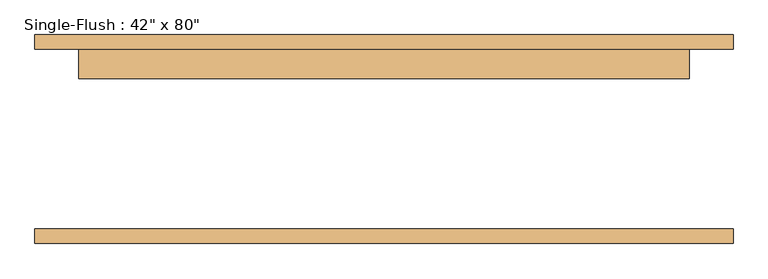
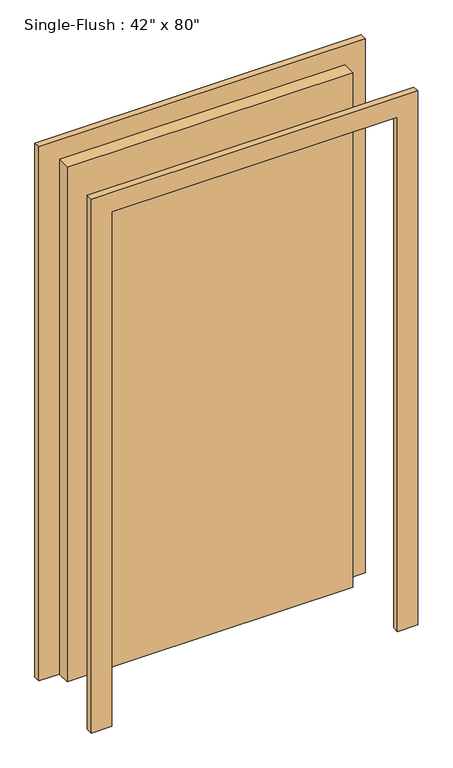
"""IFC4 building model written with IfcOpenShell, lengths in millimetres: door geometry."""

from ifc_helpers import new_model, si_unit, frame, origin, origin_with_axes, place, context, project, spatial, polyline, outline, extrude, source, transform, mapped, element, save


def door_5fd727ae(model_context):
    return source(origin(), model_context, "Body", "SweptSolid", [
        extrude(outline(polyline([(2108.2, -609.6), (0.0, -609.6), (0.0, -533.4), (2032.0, -533.4), (2032.0, 533.4), (0.0, 533.4), (0.0, 609.6), (2108.2, 609.6), (2108.2, -609.6)])), frame((0.0, 157.1625, 0.0), z_axis=(0.0, 1.0, 0.0), x_axis=(0.0, 0.0, 1.0)), (0.0, 0.0, 1.0), 25.4),
        extrude(outline(polyline([(2108.2, 609.6), (2108.2, -609.6), (0.0, -609.6), (0.0, -533.4), (2032.0, -533.4), (2032.0, 533.4), (0.0, 533.4), (0.0, 609.6), (2108.2, 609.6)])), frame((0.0, -182.5625, 0.0), z_axis=(0.0, 1.0, 0.0), x_axis=(0.0, 0.0, 1.0)), (0.0, 0.0, 1.0), 25.4),
        extrude(outline(polyline([(533.4, 106.3625), (-533.4, 106.3625), (-533.4, 157.1625), (533.4, 157.1625), (533.4, 106.3625)])), origin_with_axes(), (0.0, 0.0, 1.0), 2032.0),
    ])


if __name__ == "__main__":
    model = new_model("IFC4")
    model_context = context("Model", 3, world=origin())
    ifc_project = project(units=[si_unit("LENGTHUNIT", "METRE", prefix="MILLI")], contexts=[model_context])
    site = spatial("IfcSite", under=ifc_project)
    building = spatial("IfcBuilding", under=site)
    placement = place(None, origin())
    door_shape = door_5fd727ae(model_context)
    element("IfcDoor", 1, ObjectType="Single-Flush : 42\" x 80\"", at=placement, inside=building, context=model_context, shape_type="MappedRepresentation", body=[
        mapped(door_shape, transform((0.0, 0.0, 0.0), x_axis=(1.0, 0.0, 0.0), y_axis=(0.0, 1.0, 0.0), z_axis=(0.0, 0.0, 1.0))),
    ])
    save(model, "model.ifc")

# Revit data of these elements
# Type "Single-Flush : 42\" x 80\""
#   Type Mark = "21"
#   Construction Type Id = "MDOOR"
#   Assembly Code = "C1020"
#   Analytic Construction = "Metal"
#   Thickness = 0' - 2"
#   Heat Transfer Coefficient (U) = 3.7021 W/(m²·K)
#   Height = 6' - 8"
#   Trim Projection Ext = 0' - 1"
#   Trim Projection Int = 0' - 1"
#   Trim Width = 0' - 3"
#   Width = 3' - 6"
#   Door Material = Metal Trim
#   Frame Material = Metal Trim
#   Visual Light Transmittance = 0
#   Solar Heat Gain Coefficient = 0
#   Function = (empty or 0)
#   Wall Closure = (empty or 0)
# Element 1 (IfcDoor, "Single-Flush : 42\" x 80\"")
#   Materials on its faces: "Metal Trim"
# Materials
#   "Metal Trim": class "Wood", colour RGB 151 137 121, transparency 0, Cost = 0
